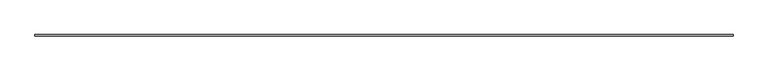
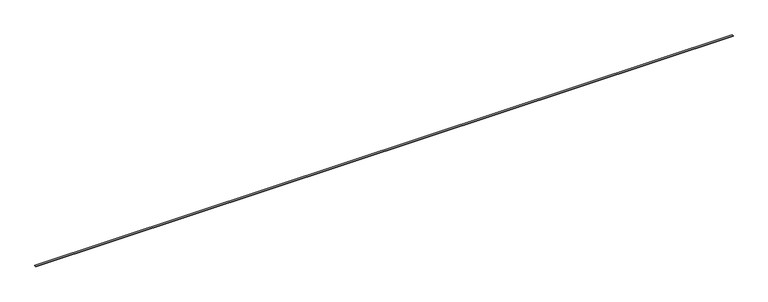
"""IFC4 building model written with IfcOpenShell, lengths in millimetres: proxy geometry, Generic Models 6:Generic Models 2:318829:Generic Models 2:318829 : Generic Models 6:Generic Models 2:318829:10 : Generic Models 6:Generic Models 2:318829:Generic Models 2:318829 : Generic Models 6:Generic Models 2:318829:300683."""

from ifc_helpers import new_model, si_unit, frame, origin, place, context, project, spatial, polyline, outline, extrude, source, transform, mapped, element, save


def generic_models_2950658e(model_context):
    return source(origin(), model_context, "Body", "SweptSolid", [
        extrude(outline(polyline([(593679.9536635, -579091.9946502), (593679.9536635, -579140.3913841), (567272.5594834, -579140.3913841), (567272.5594834, -579091.9946502), (593679.9536635, -579091.9946502)])), frame((0.0, 0.0, 2.5359006), z_axis=(0.0, 0.0, 1.0), x_axis=(1.0, 0.0, 0.0)), (0.0, 0.0, 1.0), 19.7829458),
    ])


if __name__ == "__main__":
    model = new_model("IFC4")
    model_context = context("Model", 3, world=origin())
    ifc_project = project(units=[si_unit("LENGTHUNIT", "METRE", prefix="MILLI")], contexts=[model_context])
    site = spatial("IfcSite", under=ifc_project)
    building = spatial("IfcBuilding", under=site)
    placement = place(None, origin())
    generic_models_shape = generic_models_2950658e(model_context)
    element("IfcBuildingElementProxy", 1, Name="Generic Models 6:Generic Models 2:318829:Generic Models 2:318829 : Generic Models 6:Generic Models 2:318829:10 : Generic Models 6:Generic Models 2:318829:Generic Models 2:318829 : Generic Models 6:Generic Models 2:318829:300683", ObjectType="Generic Models 6:Generic Models 2:318829:Generic Models 2:318829 : Generic Models 6:Generic Models 2:318829:10 : Generic Models 6:Generic Models 2:318829:Generic Models 2:318829 : Generic Models 6:Generic Models 2:318829:300683", at=placement, inside=building, context=model_context, shape_type="MappedRepresentation", body=[
        mapped(generic_models_shape, transform((0.0, 0.0, 0.0), x_axis=(1.0, 0.0, 0.0), y_axis=(0.0, 1.0, 0.0), z_axis=(0.0, 0.0, 1.0))),
    ])
    save(model, "model.ifc")

# Revit data of these elements
# Type "Generic Models 6:Generic Models 2:318829:Generic Models 2:318829 : Generic Models 6:Generic Models 2:318829:10 : Generic Models 6:Generic Models 2:318829:Generic Models 2:318829 : Generic Models 6:Generic Models 2:318829:300683"
#   NameOverride = "Generic Models 6:Generic Models 2:318829:Generic Models 2:318829 : Generic Models 6:Generic Models 2:318829:300683"
#   ObjectTypeOverride = "Generic Models 2:318829 : Generic Models 6:Generic Models 2:318829"
#   Reference = "Generic Models 2"
#   Tag = "300683"
# Element 1 (IfcBuildingElementProxy, "Generic Models 6:Generic Models 2:318829:Generic Models 2:318829 : Generic Models 6:Generic Models 2:318829:10 : Generic Models 6:Generic Models 2:318829:Generic Models 2:318829 : Generic Models 6:Generic Models 2:318829:300683")
#   Materials on its faces: "EXTRUDED POLYSTYRENE (XPS) RIGID FOAM INSULATION (FOAMULAR® 250 OR SIMILAR)"
# Materials
#   "EXTRUDED POLYSTYRENE (XPS) RIGID FOAM INSULATION (FOAMULAR® 250 OR SIMILAR)": class "Unassigned", colour RGB 247 185 194, transparency 0, Cost = 0
